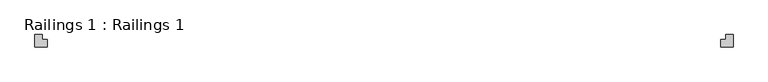
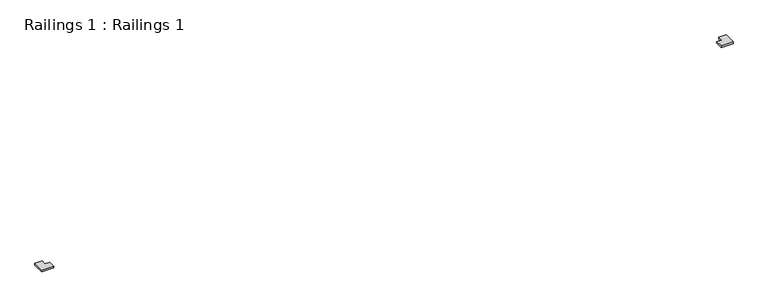
"""IFC4 building model written with IfcOpenShell, lengths in millimetres: railing geometry, Railings 1 : Railings 1."""

import ifcopenshell
import ifcopenshell.guid

model = None  # the IFC model being written
_history = None  # IfcOwnerHistory: only IFC2X3 demands one
_inside = {}  # id of a spatial element -> (the spatial element, [elements in it])
_under = {}  # id of a project, library or spatial element -> (it, [spatial elements below it])
_declared = {}  # id of a project -> (the project, [libraries it declares])
_typed = {}  # id of a type object -> (the type object, [elements of that type])
_made_of = {}  # id of a material, layer set ... -> (it, [elements and type objects made of it])


def new_model(schema):
    """Start an empty IFC model of exactly this schema.

    Asked for "IFC4X3", IfcOpenShell would pick the latest addendum, in which some entities
    have other attributes; the version numbers below select the first issue.
    IFC2X3 requires an IfcOwnerHistory on every rooted entity: one is made here for all.
    """
    global model, _history
    if schema == "IFC4X3":
        model = ifcopenshell.file(schema_version=(4, 3, 0, 0))
    else:
        model = ifcopenshell.file(schema=schema)
    _inside.clear()
    _under.clear()
    _declared.clear()
    _typed.clear()
    _made_of.clear()
    _history = None
    if model.schema == "IFC2X3":
        org = make("IfcOrganization", Name="unknown")
        user = make(
            "IfcPersonAndOrganization",
            ThePerson=make("IfcPerson", FamilyName="unknown"),
            TheOrganization=org,
        )
        app = make(
            "IfcApplication",
            ApplicationDeveloper=org,
            Version="unknown",
            ApplicationFullName="unknown",
            ApplicationIdentifier="unknown",
        )
        _history = make(
            "IfcOwnerHistory",
            OwningUser=user,
            OwningApplication=app,
            ChangeAction="ADDED",
            CreationDate=0,
        )
    return model


def make(cls, **values):
    """One entity of the class cls with the attributes given. An attribute that is None is left unset."""
    return model.create_entity(
        cls, **{name: value for name, value in values.items() if value is not None}
    )


def rooted(cls, **values):
    """An entity with a GlobalId (a new one), such as an element, a storey or a relation."""
    return make(cls, GlobalId=ifcopenshell.guid.new(), OwnerHistory=_history, **values)


def si_unit(unit_type, name, prefix=None):
    """IfcSIUnit, for example si_unit("LENGTHUNIT", "METRE", prefix="MILLI")."""
    return make("IfcSIUnit", UnitType=unit_type, Prefix=prefix, Name=name)


def assignment(units):
    """IfcUnitAssignment: the units of a project."""
    return None if units is None else make("IfcUnitAssignment", Units=units)


def point(xyz):
    """IfcCartesianPoint."""
    return None if xyz is None else make("IfcCartesianPoint", Coordinates=xyz)


def direction(xyz):
    """IfcDirection."""
    return None if xyz is None else make("IfcDirection", DirectionRatios=xyz)


def frame(location, z_axis=None, x_axis=None):
    """IfcAxis2Placement3D, a coordinate frame: its origin and axes. An axis left out is left unset."""
    return make(
        "IfcAxis2Placement3D",
        Location=point(location),
        Axis=direction(z_axis),
        RefDirection=direction(x_axis),
    )


def origin():
    """The frame at (0, 0, 0) with its axes left unset."""
    return frame((0.0, 0.0, 0.0))


def place(relative_to, where):
    """IfcLocalPlacement: puts the frame where relative to a parent placement (None: the world)."""
    return make(
        "IfcLocalPlacement", PlacementRelTo=relative_to, RelativePlacement=where
    )


def context(
    kind, dimensions, precision=None, world=None, true_north=None, identifier=None
):
    """IfcGeometricRepresentationContext, for example the 3D "Model" context."""
    return make(
        "IfcGeometricRepresentationContext",
        ContextIdentifier=identifier,
        ContextType=kind,
        CoordinateSpaceDimension=dimensions,
        Precision=precision,
        WorldCoordinateSystem=world,
        TrueNorth=true_north,
    )


def project(units=None, contexts=None):
    """IfcProject with its units and contexts."""
    return rooted(
        "IfcProject",
        Name="project",
        RepresentationContexts=contexts,
        UnitsInContext=assignment(units),
    )


def spatial(cls, under=None, at=None, **own):
    """A site, building, storey or space (cls), placed at a placement, below another one or the project."""
    s = rooted(cls, ObjectPlacement=at, **own)
    if under is not None:
        _under.setdefault(under.id(), (under, []))[1].append(s)
    return s


def polyline(points):
    """IfcPolyline through the points."""
    return make("IfcPolyline", Points=[point(p) for p in points])


def outline(outer, holes=None, kind="AREA"):
    """IfcArbitraryClosedProfileDef: a profile drawn as a closed curve; with holes, ...WithVoids."""
    if holes is None:
        return make("IfcArbitraryClosedProfileDef", ProfileType=kind, OuterCurve=outer)
    return make(
        "IfcArbitraryProfileDefWithVoids",
        ProfileType=kind,
        OuterCurve=outer,
        InnerCurves=holes,
    )


def extrude(swept, where, along, depth):
    """IfcExtrudedAreaSolid: the profile swept, set in the frame where, extruded along a direction by depth."""
    return make(
        "IfcExtrudedAreaSolid",
        SweptArea=swept,
        Position=where,
        ExtrudedDirection=direction(along),
        Depth=depth,
    )


def shape(context_of_items, identifier, shape_type, items):
    """IfcShapeRepresentation: the items that make up one representation, for example the "Body"."""
    return make(
        "IfcShapeRepresentation",
        ContextOfItems=context_of_items,
        RepresentationIdentifier=identifier,
        RepresentationType=shape_type,
        Items=items,
    )


def source(mapping_origin, context_of_items, identifier, shape_type, items):
    """IfcRepresentationMap: a shape defined once, which mapped items show again and again."""
    return make(
        "IfcRepresentationMap",
        MappingOrigin=mapping_origin,
        MappedRepresentation=shape(context_of_items, identifier, shape_type, items),
    )


def transform(
    local_origin,
    x_axis=None,
    y_axis=None,
    z_axis=None,
    scale=None,
    scale2=None,
    scale3=None,
    uniform=True,
):
    """IfcCartesianTransformationOperator3D, or its non-uniform kind. x_axis, y_axis, z_axis: its Axis1, 2, 3."""
    if uniform:
        return make(
            "IfcCartesianTransformationOperator3D",
            Axis1=direction(x_axis),
            Axis2=direction(y_axis),
            LocalOrigin=point(local_origin),
            Scale=scale,
            Axis3=direction(z_axis),
        )
    return make(
        "IfcCartesianTransformationOperator3DnonUniform",
        Axis1=direction(x_axis),
        Axis2=direction(y_axis),
        LocalOrigin=point(local_origin),
        Scale=scale,
        Axis3=direction(z_axis),
        Scale2=scale2,
        Scale3=scale3,
    )


def mapped(mapping_source, mapping_target):
    """IfcMappedItem: shows the shape of a source again, moved by a transform."""
    return make(
        "IfcMappedItem", MappingSource=mapping_source, MappingTarget=mapping_target
    )


def made_of(thing, what):
    """Note that an element or type object is made of a material, layer set ...; save() writes the relation."""
    if what is not None:
        _made_of.setdefault(what.id(), (what, []))[1].append(thing)
    return thing


def element(
    cls,
    number,
    at=None,
    inside=None,
    cuts=None,
    type_object=None,
    material=None,
    context=None,
    identifier="Body",
    shape_type=None,
    held_by="IfcProductDefinitionShape",
    body=None,
    shapes=None,
    **own,
):
    """One element of the class cls, such as IfcWall. Its Tag is "e" and its number.

    at: its placement. inside: the storey or other place that contains it. cuts: it is an
    opening in that element (IfcRelVoidsElement). A single representation is given by context,
    identifier, shape_type and body (its items); several are given by shapes. held_by: the class
    of the entity that holds the representations. save() writes the other relations.
    """
    e = rooted(cls, Tag="e%d" % number, ObjectPlacement=at, **own)
    if body is not None:
        shapes = [shape(context, identifier, shape_type, body)]
    if shapes is not None:
        e.Representation = make(held_by, Representations=shapes)
    if inside is not None:
        _inside.setdefault(inside.id(), (inside, []))[1].append(e)
    if cuts is not None:
        rooted(
            "IfcRelVoidsElement", RelatingBuildingElement=cuts, RelatedOpeningElement=e
        )
    if type_object is not None:
        _typed.setdefault(type_object.id(), (type_object, []))[1].append(e)
    return made_of(e, material)


def aggregate(whole, parts):
    """IfcRelAggregates: a whole, such as a stair, and the parts it consists of."""
    return rooted("IfcRelAggregates", RelatingObject=whole, RelatedObjects=parts)


def save(model, path):
    """Write the relations noted so far, then the file.

    IfcRelAggregates (storeys below a building ...), IfcRelContainedInSpatialStructure (elements
    in a storey), IfcRelDefinesByType, IfcRelAssociatesMaterial and IfcRelDeclares: one each for
    every whole, place, type object, material and project.
    """
    for whole, parts in _under.values():
        aggregate(whole, parts)
    for where, things in _inside.values():
        rooted(
            "IfcRelContainedInSpatialStructure",
            RelatedElements=things,
            RelatingStructure=where,
        )
    for kind, things in _typed.values():
        rooted("IfcRelDefinesByType", RelatedObjects=things, RelatingType=kind)
    for what, things in _made_of.values():
        rooted("IfcRelAssociatesMaterial", RelatedObjects=things, RelatingMaterial=what)
    for by, libraries in _declared.values():
        rooted("IfcRelDeclares", RelatingContext=by, RelatedDefinitions=libraries)
    model.write(path)


def railings_1_railings_1_7c338eaf(model_context):
    return source(origin(), model_context, "Body", "SweptSolid", [
        extrude(outline(polyline([(-1874.0398771, -3058.3548735), (-1874.0398771, -3185.4818735), (-2001.1668771, -3185.4818735), (-2001.1668771, -3109.2818735), (-1950.2398771, -3109.2818735), (-1950.2398771, -3058.3548735), (-1874.0398771, -3058.3548735)])), frame((0.0, 0.0, 4502.15), z_axis=(0.0, 0.0, 1.0), x_axis=(1.0, 0.0, 0.0)), (0.0, 0.0, 1.0), 19.05),
        extrude(outline(polyline([(-9151.2668771, -3058.3548735), (-9075.1938771, -3058.3548735), (-9075.1938771, -3109.2818735), (-9024.2668771, -3109.2818735), (-9024.2668771, -3185.4818735), (-9151.2668771, -3185.4818735), (-9151.2668771, -3058.3548735)])), frame((0.0, 0.0, 4502.15), z_axis=(0.0, 0.0, 1.0), x_axis=(1.0, 0.0, 0.0)), (0.0, 0.0, 1.0), 19.05),
    ])


if __name__ == "__main__":
    model = new_model("IFC4")
    model_context = context("Model", 3, world=origin())
    ifc_project = project(units=[si_unit("LENGTHUNIT", "METRE", prefix="MILLI")], contexts=[model_context])
    site = spatial("IfcSite", under=ifc_project)
    building = spatial("IfcBuilding", under=site)
    placement = place(None, origin())
    railings_1_railings_1_shape = railings_1_railings_1_7c338eaf(model_context)
    element("IfcRailing", 1, ObjectType="Railings 1 : Railings 1", at=placement, inside=building, context=model_context, shape_type="MappedRepresentation", body=[
        mapped(railings_1_railings_1_shape, transform((0.0, 0.0, 0.0), x_axis=(1.0, 0.0, 0.0), y_axis=(0.0, 1.0, 0.0), z_axis=(0.0, 0.0, 1.0))),
    ])
    save(model, "model.ifc")

# Revit data of these elements
# Element 1 (IfcRailing, "Railings 1 : Railings 1")
#   Materials on its faces: "Metal - Kawneer - Aluminum"
# Materials
#   "Metal - Kawneer - Aluminum": class "Metal", colour RGB 244 244 244, transparency 0, Manufacturer = "Kawneer", URL = "http://www.kawneer.com/kawneer/north_america/en/home.asp", Cost = 0
